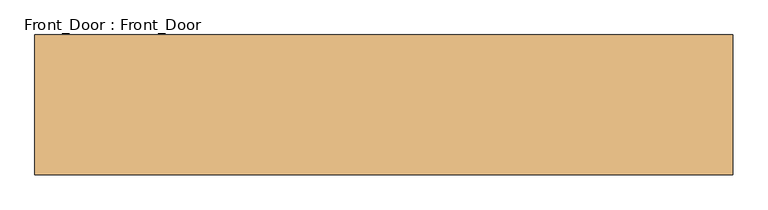
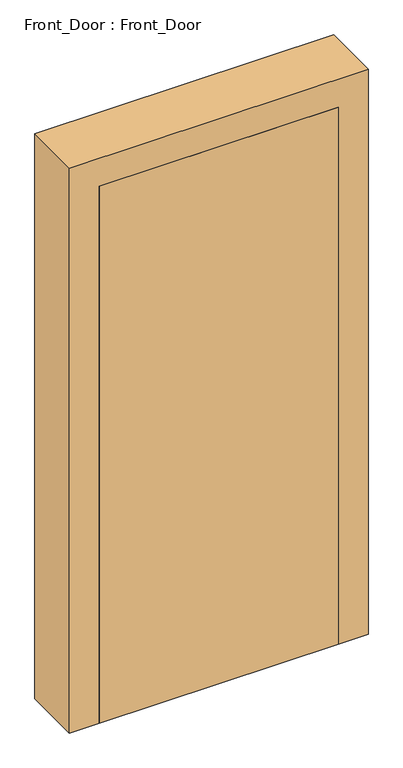
"""IFC4 building model written with IfcOpenShell, lengths in millimetres: door geometry, Front_Door : Front_Door."""

from ifc_helpers import new_model, si_unit, frame, origin, origin_with_axes, place, context, project, spatial, polyline, outline, extrude, source, transform, mapped, element, save


def front_door_front_door_f10339a7(model_context):
    return source(origin(), model_context, "Body", "SweptSolid", [
        extrude(outline(polyline([(1030.0, 445.0), (1830.0, 445.0), (1830.0, 345.0), (1030.0, 345.0), (1030.0, 445.0)])), origin_with_axes(), (0.0, 0.0, 1.0), 1900.0),
        extrude(outline(polyline([(0.0, 930.0), (0.0, 1030.0), (1900.0, 1030.0), (1900.0, 1830.0), (0.0, 1830.0), (0.0, 1930.0), (2000.0, 1930.0), (2000.0, 930.0), (0.0, 930.0)])), frame((0.0, 345.0, 0.0), z_axis=(0.0, 1.0, 0.0), x_axis=(0.0, 0.0, 1.0)), (0.0, 0.0, 1.0), 200.0),
    ])


if __name__ == "__main__":
    model = new_model("IFC4")
    model_context = context("Model", 3, world=origin())
    ifc_project = project(units=[si_unit("LENGTHUNIT", "METRE", prefix="MILLI")], contexts=[model_context])
    site = spatial("IfcSite", under=ifc_project)
    building = spatial("IfcBuilding", under=site)
    placement = place(None, origin())
    front_door_front_door_shape = front_door_front_door_f10339a7(model_context)
    element("IfcDoor", 1, ObjectType="Front_Door : Front_Door", at=placement, inside=building, context=model_context, shape_type="MappedRepresentation", body=[
        mapped(front_door_front_door_shape, transform((0.0, 0.0, 0.0), x_axis=(1.0, 0.0, 0.0), y_axis=(0.0, 1.0, 0.0), z_axis=(0.0, 0.0, 1.0))),
    ])
    save(model, "model.ifc")

# Revit data of these elements
# Type "Front_Door : Front_Door"
#   Type Mark = "47"
#   NameOverride = "Front_Door"
# Element 1 (IfcDoor, "Front_Door : Front_Door")
#   Materials on its faces: "IfcSurfaceStyle #392"
# Materials
#   "IfcSurfaceStyle #392": class "Unassigned", colour RGB 204 204 204, transparency 0
